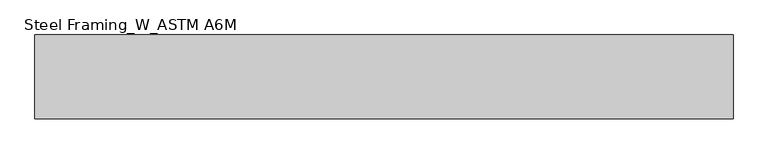
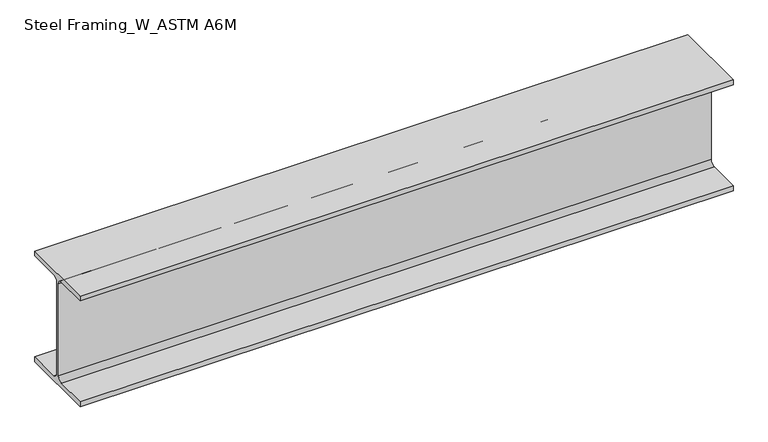
"""IFC4 building model written with IfcOpenShell, lengths in millimetres: beam geometry, Steel Framing_W_ASTM A6M : H_SB_AR_S02_W310x60_B5."""

from ifc_helpers import new_model, si_unit, point, frame, frame_2d, origin, place, context, project, spatial, polyline, circle_curve, trimmed, segment, composite_curve, outline, extrude, source, transform, mapped, element, save


def steel_framing_w_astm_a6m_1b89ef3a(model_context):
    return source(origin(), model_context, "Body", "SweptSolid", [
        extrude(outline(composite_curve([segment(polyline([(101.5, -137.9), (101.5, -151.0), (-101.5, -151.0), (-101.5, -137.9), (-16.545, -137.9)]), True, "CONTINUOUS"), segment(trimmed(circle_curve(frame_2d((-16.545, -125.1)), 12.8), [point((-16.545, -137.9))], [point((-3.745, -125.1))], True, "CARTESIAN"), True, "CONTINUOUS"), segment(polyline([(-3.745, -125.1), (-3.745, 125.1)]), True, "CONTINUOUS"), segment(trimmed(circle_curve(frame_2d((-16.545, 125.1)), 12.8), [point((-3.745, 125.1))], [point((-16.545, 137.9))], True, "CARTESIAN"), True, "CONTINUOUS"), segment(polyline([(-16.545, 137.9), (-101.5, 137.9), (-101.5, 151.0), (101.5, 151.0), (101.5, 137.9), (16.545, 137.9)]), True, "CONTINUOUS"), segment(trimmed(circle_curve(frame_2d((16.545, 125.1)), 12.8), [point((16.545, 137.9))], [point((3.745, 125.1))], True, "CARTESIAN"), True, "CONTINUOUS"), segment(polyline([(3.745, 125.1), (3.745, -125.1)]), True, "CONTINUOUS"), segment(trimmed(circle_curve(frame_2d((16.545, -125.1)), 12.8), [point((3.745, -125.1))], [point((16.545, -137.9))], True, "CARTESIAN"), True, "CONTINUOUS"), segment(polyline([(16.545, -137.9), (101.5, -137.9)]), True, "CONTINUOUS")], self_intersect=False)), frame((-735.3, 0.0, 0.0), z_axis=(1.0, 0.0, 0.0), x_axis=(0.0, 1.0, 0.0)), (0.0, 0.0, 1.0), 1686.8),
    ])


if __name__ == "__main__":
    model = new_model("IFC4")
    model_context = context("Model", 3, world=origin())
    ifc_project = project(units=[si_unit("LENGTHUNIT", "METRE", prefix="MILLI")], contexts=[model_context])
    site = spatial("IfcSite", under=ifc_project)
    building = spatial("IfcBuilding", under=site)
    placement = place(None, origin())
    steel_framing_w_astm_a6m_shape = steel_framing_w_astm_a6m_1b89ef3a(model_context)
    element("IfcBeam", 1, ObjectType="Steel Framing_W_ASTM A6M : H_SB_AR_S02_W310x60_B5", at=placement, inside=building, context=model_context, shape_type="MappedRepresentation", body=[
        mapped(steel_framing_w_astm_a6m_shape, transform((0.0, 0.0, 0.0), x_axis=(1.0, 0.0, 0.0), y_axis=(0.0, 1.0, 0.0), z_axis=(0.0, 0.0, 1.0))),
    ])
    save(model, "model.ifc")

# Revit data of these elements
# Type "Steel Framing_W_ASTM A6M : H_SB_AR_S02_W310x60_B5"
#   Type Mark = "B5"
#   Section Name Key = "W12x40"
#   Width = 20.3 cm
#   Web Thickness = 0.749 cm
#   Web Fillet = 1.28 cm
#   Warping Constant = 387000.0 cm⁶
#   Torsional Moment of Inertia = 37.70 cm⁴
#   Section Area = 75.5 cm²
#   Plastic Modulus weak axis = 275.0 cm³
#   Plastic Modulus strong axis = 934.0 cm³
#   Perimeter = 1.38 m²/m
#   Nominal Weight = 60.00 kgf/m
#   Moment of Inertia weak axis = 1840.00 cm⁴
#   Moment of Inertia strong axis = 12800.00 cm⁴
#   Height = 30.2 cm
#   Flange Thickness = 1.31 cm
#   Elastic Modulus weak axis = 180.0 cm³
#   Elastic Modulus strong axis = 844.0 cm³
#   Centroid Vertical = 15.1 cm
#   Centroid Horizontal = 10.15 cm
#   Length [instance default] = 1500 mm
#   Structural Material [instance default] = Steel, 45-345
#   Bolt Spacing = 0
#   Assembly Code = ""
# Element 1 (IfcBeam, "Steel Framing_W_ASTM A6M : H_SB_AR_S02_W310x60_B5")
#   Materials on its faces: "Steel, 45-345"
# Materials
#   "Steel, 45-345": class "Metal", colour RGB 189 187 185, transparency 0, Description = "Steel 345 MPa", Cost = 0
